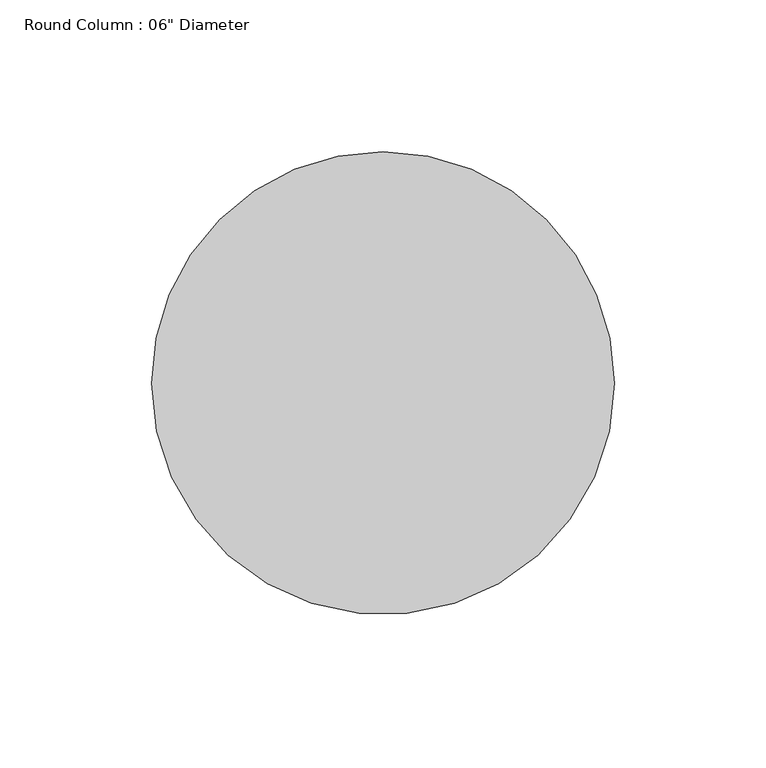
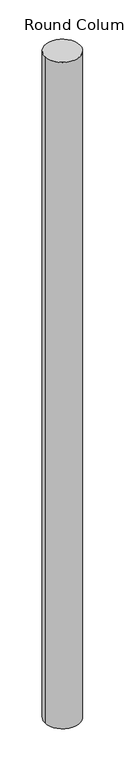
"""IFC4 building model written with IfcOpenShell, lengths in millimetres: column geometry."""

import ifcopenshell
import ifcopenshell.guid

model = None  # the IFC model being written
_history = None  # IfcOwnerHistory: only IFC2X3 demands one
_inside = {}  # id of a spatial element -> (the spatial element, [elements in it])
_under = {}  # id of a project, library or spatial element -> (it, [spatial elements below it])
_declared = {}  # id of a project -> (the project, [libraries it declares])
_typed = {}  # id of a type object -> (the type object, [elements of that type])
_made_of = {}  # id of a material, layer set ... -> (it, [elements and type objects made of it])


def new_model(schema):
    """Start an empty IFC model of exactly this schema.

    Asked for "IFC4X3", IfcOpenShell would pick the latest addendum, in which some entities
    have other attributes; the version numbers below select the first issue.
    IFC2X3 requires an IfcOwnerHistory on every rooted entity: one is made here for all.
    """
    global model, _history
    if schema == "IFC4X3":
        model = ifcopenshell.file(schema_version=(4, 3, 0, 0))
    else:
        model = ifcopenshell.file(schema=schema)
    _inside.clear()
    _under.clear()
    _declared.clear()
    _typed.clear()
    _made_of.clear()
    _history = None
    if model.schema == "IFC2X3":
        org = make("IfcOrganization", Name="unknown")
        user = make(
            "IfcPersonAndOrganization",
            ThePerson=make("IfcPerson", FamilyName="unknown"),
            TheOrganization=org,
        )
        app = make(
            "IfcApplication",
            ApplicationDeveloper=org,
            Version="unknown",
            ApplicationFullName="unknown",
            ApplicationIdentifier="unknown",
        )
        _history = make(
            "IfcOwnerHistory",
            OwningUser=user,
            OwningApplication=app,
            ChangeAction="ADDED",
            CreationDate=0,
        )
    return model


def make(cls, **values):
    """One entity of the class cls with the attributes given. An attribute that is None is left unset."""
    return model.create_entity(
        cls, **{name: value for name, value in values.items() if value is not None}
    )


def rooted(cls, **values):
    """An entity with a GlobalId (a new one), such as an element, a storey or a relation."""
    return make(cls, GlobalId=ifcopenshell.guid.new(), OwnerHistory=_history, **values)


def si_unit(unit_type, name, prefix=None):
    """IfcSIUnit, for example si_unit("LENGTHUNIT", "METRE", prefix="MILLI")."""
    return make("IfcSIUnit", UnitType=unit_type, Prefix=prefix, Name=name)


def assignment(units):
    """IfcUnitAssignment: the units of a project."""
    return None if units is None else make("IfcUnitAssignment", Units=units)


def point(xyz):
    """IfcCartesianPoint."""
    return None if xyz is None else make("IfcCartesianPoint", Coordinates=xyz)


def direction(xyz):
    """IfcDirection."""
    return None if xyz is None else make("IfcDirection", DirectionRatios=xyz)


def frame(location, z_axis=None, x_axis=None):
    """IfcAxis2Placement3D, a coordinate frame: its origin and axes. An axis left out is left unset."""
    return make(
        "IfcAxis2Placement3D",
        Location=point(location),
        Axis=direction(z_axis),
        RefDirection=direction(x_axis),
    )


def frame_2d(location, x_axis=None):
    """IfcAxis2Placement2D, a coordinate frame in the plane: its origin and x axis."""
    return make(
        "IfcAxis2Placement2D", Location=point(location), RefDirection=direction(x_axis)
    )


def origin():
    """The frame at (0, 0, 0) with its axes left unset."""
    return frame((0.0, 0.0, 0.0))


def origin_with_axes():
    """The frame at (0, 0, 0) with the z axis (0, 0, 1) and the x axis (1, 0, 0) written out."""
    return frame((0.0, 0.0, 0.0), z_axis=(0.0, 0.0, 1.0), x_axis=(1.0, 0.0, 0.0))


def origin_2d():
    """The frame at (0, 0) in the plane with its x axis left unset."""
    return frame_2d((0.0, 0.0))


def place(relative_to, where):
    """IfcLocalPlacement: puts the frame where relative to a parent placement (None: the world)."""
    return make(
        "IfcLocalPlacement", PlacementRelTo=relative_to, RelativePlacement=where
    )


def context(
    kind, dimensions, precision=None, world=None, true_north=None, identifier=None
):
    """IfcGeometricRepresentationContext, for example the 3D "Model" context."""
    return make(
        "IfcGeometricRepresentationContext",
        ContextIdentifier=identifier,
        ContextType=kind,
        CoordinateSpaceDimension=dimensions,
        Precision=precision,
        WorldCoordinateSystem=world,
        TrueNorth=true_north,
    )


def project(units=None, contexts=None):
    """IfcProject with its units and contexts."""
    return rooted(
        "IfcProject",
        Name="project",
        RepresentationContexts=contexts,
        UnitsInContext=assignment(units),
    )


def spatial(cls, under=None, at=None, **own):
    """A site, building, storey or space (cls), placed at a placement, below another one or the project."""
    s = rooted(cls, ObjectPlacement=at, **own)
    if under is not None:
        _under.setdefault(under.id(), (under, []))[1].append(s)
    return s


def circle_curve(where, radius):
    """IfcCircle in the frame where."""
    return make("IfcCircle", Position=where, Radius=radius)


def trimmed(basis, trim1, trim2, sense, master):
    """IfcTrimmedCurve: the piece of a basis curve between two trims."""
    return make(
        "IfcTrimmedCurve",
        BasisCurve=basis,
        Trim1=trim1,
        Trim2=trim2,
        SenseAgreement=sense,
        MasterRepresentation=master,
    )


def segment(curve, same_sense, transition):
    """IfcCompositeCurveSegment."""
    return make(
        "IfcCompositeCurveSegment",
        Transition=transition,
        SameSense=same_sense,
        ParentCurve=curve,
    )


def composite_curve(segments, self_intersect=None):
    """IfcCompositeCurve: segments joined end to end."""
    return make("IfcCompositeCurve", Segments=segments, SelfIntersect=self_intersect)


def outline(outer, holes=None, kind="AREA"):
    """IfcArbitraryClosedProfileDef: a profile drawn as a closed curve; with holes, ...WithVoids."""
    if holes is None:
        return make("IfcArbitraryClosedProfileDef", ProfileType=kind, OuterCurve=outer)
    return make(
        "IfcArbitraryProfileDefWithVoids",
        ProfileType=kind,
        OuterCurve=outer,
        InnerCurves=holes,
    )


def extrude(swept, where, along, depth):
    """IfcExtrudedAreaSolid: the profile swept, set in the frame where, extruded along a direction by depth."""
    return make(
        "IfcExtrudedAreaSolid",
        SweptArea=swept,
        Position=where,
        ExtrudedDirection=direction(along),
        Depth=depth,
    )


def shape(context_of_items, identifier, shape_type, items):
    """IfcShapeRepresentation: the items that make up one representation, for example the "Body"."""
    return make(
        "IfcShapeRepresentation",
        ContextOfItems=context_of_items,
        RepresentationIdentifier=identifier,
        RepresentationType=shape_type,
        Items=items,
    )


def source(mapping_origin, context_of_items, identifier, shape_type, items):
    """IfcRepresentationMap: a shape defined once, which mapped items show again and again."""
    return make(
        "IfcRepresentationMap",
        MappingOrigin=mapping_origin,
        MappedRepresentation=shape(context_of_items, identifier, shape_type, items),
    )


def transform(
    local_origin,
    x_axis=None,
    y_axis=None,
    z_axis=None,
    scale=None,
    scale2=None,
    scale3=None,
    uniform=True,
):
    """IfcCartesianTransformationOperator3D, or its non-uniform kind. x_axis, y_axis, z_axis: its Axis1, 2, 3."""
    if uniform:
        return make(
            "IfcCartesianTransformationOperator3D",
            Axis1=direction(x_axis),
            Axis2=direction(y_axis),
            LocalOrigin=point(local_origin),
            Scale=scale,
            Axis3=direction(z_axis),
        )
    return make(
        "IfcCartesianTransformationOperator3DnonUniform",
        Axis1=direction(x_axis),
        Axis2=direction(y_axis),
        LocalOrigin=point(local_origin),
        Scale=scale,
        Axis3=direction(z_axis),
        Scale2=scale2,
        Scale3=scale3,
    )


def mapped(mapping_source, mapping_target):
    """IfcMappedItem: shows the shape of a source again, moved by a transform."""
    return make(
        "IfcMappedItem", MappingSource=mapping_source, MappingTarget=mapping_target
    )


def made_of(thing, what):
    """Note that an element or type object is made of a material, layer set ...; save() writes the relation."""
    if what is not None:
        _made_of.setdefault(what.id(), (what, []))[1].append(thing)
    return thing


def element(
    cls,
    number,
    at=None,
    inside=None,
    cuts=None,
    type_object=None,
    material=None,
    context=None,
    identifier="Body",
    shape_type=None,
    held_by="IfcProductDefinitionShape",
    body=None,
    shapes=None,
    **own,
):
    """One element of the class cls, such as IfcWall. Its Tag is "e" and its number.

    at: its placement. inside: the storey or other place that contains it. cuts: it is an
    opening in that element (IfcRelVoidsElement). A single representation is given by context,
    identifier, shape_type and body (its items); several are given by shapes. held_by: the class
    of the entity that holds the representations. save() writes the other relations.
    """
    e = rooted(cls, Tag="e%d" % number, ObjectPlacement=at, **own)
    if body is not None:
        shapes = [shape(context, identifier, shape_type, body)]
    if shapes is not None:
        e.Representation = make(held_by, Representations=shapes)
    if inside is not None:
        _inside.setdefault(inside.id(), (inside, []))[1].append(e)
    if cuts is not None:
        rooted(
            "IfcRelVoidsElement", RelatingBuildingElement=cuts, RelatedOpeningElement=e
        )
    if type_object is not None:
        _typed.setdefault(type_object.id(), (type_object, []))[1].append(e)
    return made_of(e, material)


def aggregate(whole, parts):
    """IfcRelAggregates: a whole, such as a stair, and the parts it consists of."""
    return rooted("IfcRelAggregates", RelatingObject=whole, RelatedObjects=parts)


def save(model, path):
    """Write the relations noted so far, then the file.

    IfcRelAggregates (storeys below a building ...), IfcRelContainedInSpatialStructure (elements
    in a storey), IfcRelDefinesByType, IfcRelAssociatesMaterial and IfcRelDeclares: one each for
    every whole, place, type object, material and project.
    """
    for whole, parts in _under.values():
        aggregate(whole, parts)
    for where, things in _inside.values():
        rooted(
            "IfcRelContainedInSpatialStructure",
            RelatedElements=things,
            RelatingStructure=where,
        )
    for kind, things in _typed.values():
        rooted("IfcRelDefinesByType", RelatedObjects=things, RelatingType=kind)
    for what, things in _made_of.values():
        rooted("IfcRelAssociatesMaterial", RelatedObjects=things, RelatingMaterial=what)
    for by, libraries in _declared.values():
        rooted("IfcRelDeclares", RelatingContext=by, RelatedDefinitions=libraries)
    model.write(path)


def column_79e7fb11(model_context):
    return source(origin(), model_context, "Body", "SweptSolid", [
        extrude(outline(composite_curve([segment(trimmed(circle_curve(origin_2d(), 76.2), [point((76.2, 0.0))], [point((-76.2, 0.0))], False, "CARTESIAN"), True, "CONTINUOUS"), segment(trimmed(circle_curve(origin_2d(), 76.2), [point((-76.2, 0.0))], [point((0.0, 76.2))], False, "CARTESIAN"), True, "CONTINUOUS"), segment(trimmed(circle_curve(origin_2d(), 76.2), [point((0.0, 76.2))], [point((76.2, 0.0))], False, "CARTESIAN"), True, "CONTINUOUS")], self_intersect=False)), origin_with_axes(), (0.0, 0.0, 1.0), 3048.0),
    ])


if __name__ == "__main__":
    model = new_model("IFC4")
    model_context = context("Model", 3, world=origin())
    ifc_project = project(units=[si_unit("LENGTHUNIT", "METRE", prefix="MILLI")], contexts=[model_context])
    site = spatial("IfcSite", under=ifc_project)
    building = spatial("IfcBuilding", under=site)
    placement = place(None, origin())
    column_shape = column_79e7fb11(model_context)
    element("IfcColumn", 1, ObjectType="Round Column : 06\" Diameter", at=placement, inside=building, context=model_context, shape_type="MappedRepresentation", body=[
        mapped(column_shape, transform((0.0, 0.0, 0.0), x_axis=(1.0, 0.0, 0.0), y_axis=(0.0, 1.0, 0.0), z_axis=(0.0, 0.0, 1.0))),
    ])
    save(model, "model.ifc")

# Revit data of these elements
# Type "Round Column : 06\" Diameter"
#   Assembly Code = "B1010200"
#   Diameter = 0' - 6"
#   Offset Base = 0' - 0"
#   Offset Top = 0' - 0"
#   Material = Wood - Cherry
# Element 1 (IfcColumn, "Round Column : 06\" Diameter")
#   Materials on its faces: "Wood - Cherry"
# Materials
#   "Wood - Cherry": class "Unassigned", colour RGB 226 177 128, transparency 0
